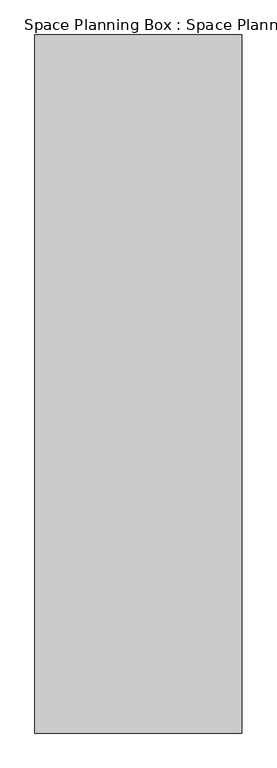
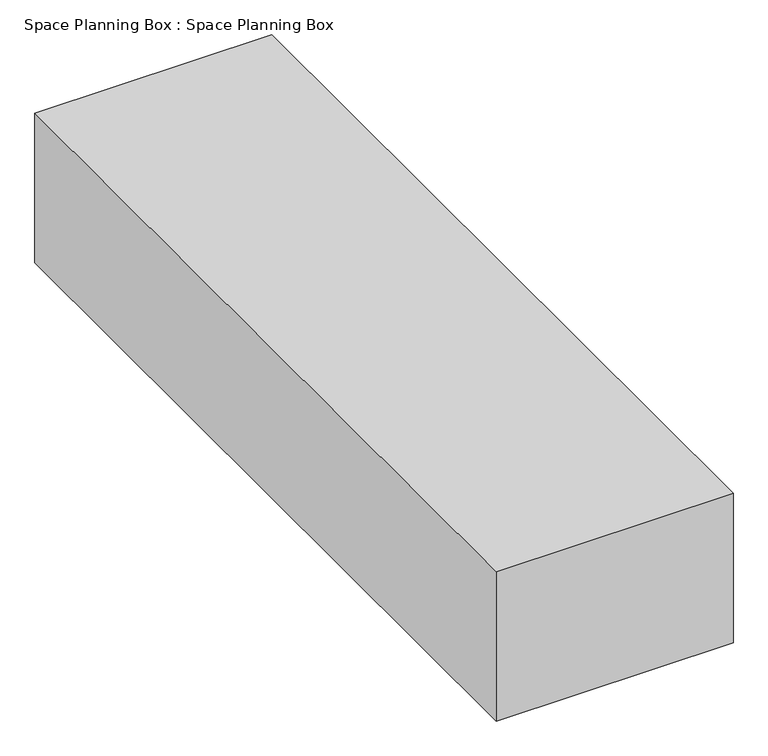
"""IFC4 building model written with IfcOpenShell, lengths in millimetres: proxy geometry, Space Planning Box : Space Planning Box."""

from ifc_helpers import new_model, si_unit, origin, origin_with_axes, place, context, project, spatial, polyline, outline, extrude, source, transform, mapped, element, save


def space_planning_box_space_planning_box_ce7d2093(model_context):
    return source(origin(), model_context, "Body", "SweptSolid", [
        extrude(outline(polyline([(4500.0, 15175.0), (4500.0, -15175.0), (-4500.0, -15175.0), (-4500.0, 15175.0), (4500.0, 15175.0)])), origin_with_axes(), (0.0, 0.0, 1.0), 6000.0),
    ])


if __name__ == "__main__":
    model = new_model("IFC4")
    model_context = context("Model", 3, world=origin())
    ifc_project = project(units=[si_unit("LENGTHUNIT", "METRE", prefix="MILLI")], contexts=[model_context])
    site = spatial("IfcSite", under=ifc_project)
    building = spatial("IfcBuilding", under=site)
    placement = place(None, origin())
    space_planning_box_space_planning_box_shape = space_planning_box_space_planning_box_ce7d2093(model_context)
    element("IfcBuildingElementProxy", 1, Name="Space Planning Box : Space Planning Box", ObjectType="Space Planning Box : Space Planning Box", at=placement, inside=building, context=model_context, shape_type="MappedRepresentation", body=[
        mapped(space_planning_box_space_planning_box_shape, transform((0.0, 0.0, 0.0), x_axis=(1.0, 0.0, 0.0), y_axis=(0.0, 1.0, 0.0), z_axis=(0.0, 0.0, 1.0))),
    ])
    save(model, "model.ifc")

# Revit data of these elements
# Type "Space Planning Box : Space Planning Box"
#   Type Comments = "..."
#   Room Name [instance default] = "?"
#   Assembly Code = "..."
#   Width [instance default] = 1524 mm
#   Program Area [instance default] = 0 m²
#   Length [instance default] = 1524 mm
#   Height [instance default] = 1524 mm
#   Area [instance default] = 2.32258 m²
#   Fill Color [instance default] = Cyan
#   Default Elevation = 0
# Element 1 (IfcBuildingElementProxy, "Space Planning Box : Space Planning Box")
#   Room Name = "Central Control Room"
#   Width = 9000 mm
#   Program Area = 288 m²
#   Length = 30350 mm
#   Height = 6000 mm
#   Area = 273.15 m²
#   Fill Color = Lime
#   Materials on its faces: "Lime"
# Materials
#   "Cyan": class "Generic", colour RGB 0 255 255, transparency 0.2, Cost = 0
#   "Lime": class "Generic", colour RGB 0 255 0, transparency 0.2, Cost = 0
